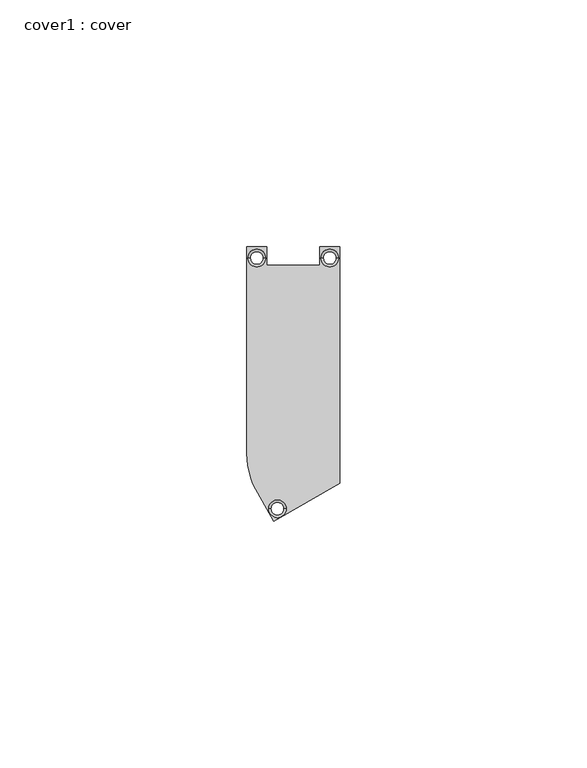
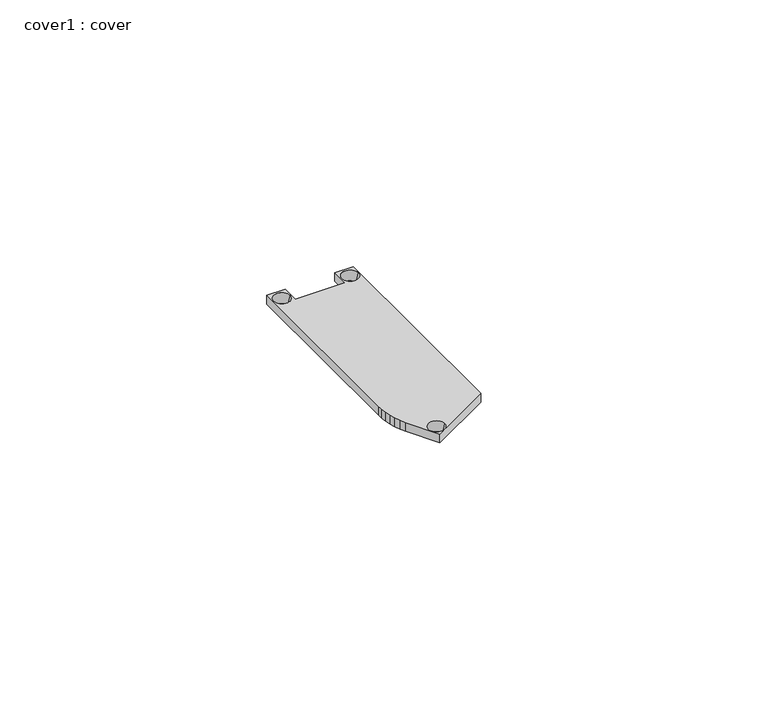
"""IFC4 building model written with IfcOpenShell, lengths in millimetres: proxy geometry, cover1 : cover."""

from ifc_helpers import new_model, si_unit, frame, origin, place, context, project, spatial, polyline, circle_curve, source, transform, mapped, element, save
from ifc_brep_helpers import plane_surface, revolved_surface, advanced_brep


def cover1_cover_a61f0212(model_context):
    return source(origin(), model_context, "Body", "AdvancedBrep", [
        advanced_brep(
        [(4738.4618953, 3578.6670305, 2.0), (4734.4613953, 3578.6670305, 2.0), (4734.4613953, 3574.9179905, 2.0), (4723.6816353, 3574.9179905, 2.0), (4723.6816353, 3578.6670305, 2.0), (4719.6811353, 3578.6670305, 2.0), (4719.6811353, 3536.8840305, 2.0), (4719.7370153, 3535.6191105, 2.0), (4719.8919553, 3534.3618105, 2.0), (4720.1383353, 3533.1222905, 2.0), (4720.4786953, 3531.9030905, 2.0), (4720.9079553, 3530.7118305, 2.0), (4721.4261153, 3529.5586705, 2.0), (4725.1243775, 3523.1530364, 2.0), (4738.4618953, 3530.8564939, 2.0), (4738.2616453, 3576.4165905, 2.0), (4734.6616453, 3576.4165905, 2.0), (4723.4801153, 3576.4165905, 2.0), (4719.8801153, 3576.4165905, 2.0), (4727.6343594, 3525.6369105, 2.0), (4724.0799311, 3525.6369105, 2.0), (4738.4618953, 3578.6670305, 0.0), (4738.4618953, 3530.8564939, 0.0), (4725.1243775, 3523.1530364, 0.0), (4721.4261153, 3529.5586705, 0.0), (4720.9079553, 3530.7118305, 0.0), (4720.4786953, 3531.9030905, 0.0), (4720.1383353, 3533.1222905, 0.0), (4719.8919553, 3534.3618105, 0.0), (4719.7370153, 3535.6191105, 0.0), (4719.6811353, 3536.8840305, 0.0), (4719.6811353, 3578.6670305, 0.0), (4723.6816353, 3578.6670305, 0.0), (4723.6816353, 3574.9179905, 0.0), (4734.4613953, 3574.9179905, 0.0), (4734.4613953, 3578.6670305, 0.0), (4735.1616453, 3576.4165905, 0.0), (4737.7616453, 3576.4165905, 0.0), (4720.3801153, 3576.4165905, 0.0), (4722.9801153, 3576.4165905, 0.0), (4724.5418919, 3525.6369105, 0.0), (4727.1723986, 3525.6369105, 0.0)],
        [
            (0, 1),
            (1, 2),
            (2, 3),
            (3, 4),
            (4, 5),
            (5, 6),
            (6, 7),
            (7, 8),
            (8, 9),
            (9, 10),
            (10, 11),
            (11, 12),
            (12, 13),
            (13, 14),
            (14, 0),
            (15, 16, circle_curve(frame((4736.4616453, 3576.4165905, 2.0), z_axis=(0.0, 0.0, -1.0), x_axis=(-1.0, 0.0, 0.0)), 1.8)),
            (16, 15, circle_curve(frame((4736.4616453, 3576.4165905, 2.0), z_axis=(0.0, 0.0, -1.0), x_axis=(1.0, 0.0, 0.0)), 1.8)),
            (17, 18, circle_curve(frame((4721.6801153, 3576.4165905, 2.0), z_axis=(0.0, 0.0, -1.0), x_axis=(-1.0, 0.0, 0.0)), 1.8)),
            (18, 17, circle_curve(frame((4721.6801153, 3576.4165905, 2.0), z_axis=(0.0, 0.0, -1.0), x_axis=(1.0, 0.0, 0.0)), 1.8)),
            (19, 20, circle_curve(frame((4725.8571453, 3525.6369105, 2.0), z_axis=(0.0, 0.0, -1.0), x_axis=(-1.0, 0.0, 0.0)), 1.7772142)),
            (20, 19, circle_curve(frame((4725.8571453, 3525.6369105, 2.0), z_axis=(0.0, 0.0, -1.0), x_axis=(1.0, 0.0, 0.0)), 1.7772142)),
            (21, 22),
            (22, 23),
            (23, 24),
            (24, 25),
            (25, 26),
            (26, 27),
            (27, 28),
            (28, 29),
            (29, 30),
            (30, 31),
            (31, 32),
            (32, 33),
            (33, 34),
            (34, 35),
            (35, 21),
            (36, 37, circle_curve(frame((4736.4616453, 3576.4165905, 0.0), z_axis=(0.0, 0.0, 1.0), x_axis=(-1.0, 0.0, 0.0)), 1.3)),
            (37, 36, circle_curve(frame((4736.4616453, 3576.4165905, 0.0), z_axis=(0.0, 0.0, 1.0), x_axis=(1.0, 0.0, 0.0)), 1.3)),
            (38, 39, circle_curve(frame((4721.6801153, 3576.4165905, 0.0), z_axis=(0.0, 0.0, 1.0), x_axis=(-1.0, 0.0, 0.0)), 1.3)),
            (39, 38, circle_curve(frame((4721.6801153, 3576.4165905, 0.0), z_axis=(0.0, 0.0, 1.0), x_axis=(1.0, 0.0, 0.0)), 1.3)),
            (40, 41, circle_curve(frame((4725.8571453, 3525.6369105, 0.0), z_axis=(0.0, 0.0, 1.0), x_axis=(-1.0, 0.0, 0.0)), 1.3152534)),
            (41, 40, circle_curve(frame((4725.8571453, 3525.6369105, 0.0), z_axis=(0.0, 0.0, 1.0), x_axis=(1.0, 0.0, 0.0)), 1.3152534)),
            (14, 22),
            (21, 0),
            (13, 23),
            (12, 24),
            (5, 31),
            (30, 6),
            (11, 25),
            (10, 26),
            (9, 27),
            (8, 28),
            (7, 29),
            (4, 32),
            (36, 16),
            (15, 37),
            (38, 18),
            (17, 39),
            (40, 20),
            (19, 41),
            (3, 33),
            (2, 34),
            (1, 35),
        ],
        [
            plane_surface(frame((4734.4613953, 3578.6670305, 2.0), z_axis=(0.0, 0.0, 1.0), x_axis=(-1.0, 0.0, 0.0))),
            plane_surface(frame((4734.4613953, 3578.6670305, 0.0), z_axis=(0.0, 0.0, -1.0), x_axis=(1.0, 0.0, 0.0))),
            plane_surface(frame((4738.4618953, 3530.8564939, 2.0), z_axis=(1.0, 0.0, 0.0), x_axis=(0.0, 0.0, -1.0))),
            plane_surface(frame((4725.1243775, 3523.1530364, 2.0), z_axis=(0.5001479267947538, -0.8659399813629751, 0.0), x_axis=(0.0, 0.0, -1.0))),
            plane_surface(frame((4721.4261153, 3529.5586705, 2.0), z_axis=(-0.8660272939548952, -0.49999672611444335, 0.0), x_axis=(0.0, 0.0, -1.0))),
            plane_surface(frame((4719.6811353, 3578.6670305, 2.0), z_axis=(-1.0, 0.0, 0.0), x_axis=(0.0, 0.0, -1.0))),
            plane_surface(frame((4720.9079553, 3530.7118305, 2.0), z_axis=(-0.91214692510674, -0.40986337603928397, 0.0), x_axis=(0.0, 0.0, -1.0))),
            plane_surface(frame((4720.4786953, 3531.9030905, 2.0), z_axis=(-0.9407850831608502, -0.3390035800725891, 0.0), x_axis=(0.0, 0.0, -1.0))),
            plane_surface(frame((4720.1383353, 3533.1222905, 2.0), z_axis=(-0.9631721335643817, -0.26888555395379093, 0.0), x_axis=(0.0, 0.0, -1.0))),
            plane_surface(frame((4719.8919553, 3534.3618105, 2.0), z_axis=(-0.9808118970912181, -0.19495646315094542, 0.0), x_axis=(0.0, 0.0, -1.0))),
            plane_surface(frame((4719.7370153, 3535.6191105, 2.0), z_axis=(-0.9924922999614717, -0.12230713191465294, 0.0), x_axis=(0.0, 0.0, -1.0))),
            plane_surface(frame((4719.6811353, 3536.8840305, 2.0), z_axis=(-0.9990256352193916, -0.04413366260000536, 0.0), x_axis=(0.0, 0.0, -1.0))),
            plane_surface(frame((4723.6816353, 3578.6670305, 2.0), z_axis=(0.0, 1.0, 0.0), x_axis=(0.0, 0.0, -1.0))),
            revolved_surface(polyline([(4734.6616453, 3576.4165905, 2.0), (4735.1616453, 3576.4165905, 0.0)]), (4736.4616453, 3576.4165905, -5.2), (0.0, 0.0, 1.0)),
            revolved_surface(polyline([(4719.8801153, 3576.4165905, 2.0), (4720.3801153, 3576.4165905, 0.0)]), (4721.6801153, 3576.4165905, -5.2), (0.0, 0.0, 1.0)),
            revolved_surface(polyline([(4724.0799311, 3525.6369105, 2.0), (4724.5418919125095, 3525.6369105, 0.0)]), (4725.8571453, 3525.6369105, -5.6942206), (0.0, 0.0, 1.0)),
            plane_surface(frame((4723.6816353, 3574.9179905, 2.0), z_axis=(1.0, 0.0, 0.0), x_axis=(0.0, 0.0, -1.0))),
            plane_surface(frame((4734.4613953, 3574.9179905, 2.0), z_axis=(0.0, 1.0, 0.0), x_axis=(0.0, 0.0, -1.0))),
            plane_surface(frame((4734.4613953, 3578.6670305, 2.0), z_axis=(-1.0, 0.0, 0.0), x_axis=(0.0, 0.0, -1.0))),
            plane_surface(frame((4738.4618953, 3578.6670305, 2.0), z_axis=(0.0, 1.0, 0.0), x_axis=(0.0, 0.0, -1.0))),
        ],
        [
            (0, [[1, 2, 3, 4, 5, 6, 7, 8, 9, 10, 11, 12, 13, 14, 15], [16, 17], [18, 19], [20, 21]]),
            (1, [[22, 23, 24, 25, 26, 27, 28, 29, 30, 31, 32, 33, 34, 35, 36], [37, 38], [39, 40], [41, 42]]),
            (2, [[-15, 43, -22, 44]]),
            (3, [[-14, 45, -23, -43]]),
            (4, [[-13, 46, -24, -45]]),
            (5, [[-6, 47, -31, 48]]),
            (6, [[-12, 49, -25, -46]]),
            (7, [[-11, 50, -26, -49]]),
            (8, [[-10, 51, -27, -50]]),
            (9, [[-9, 52, -28, -51]]),
            (10, [[-8, 53, -29, -52]]),
            (11, [[-7, -48, -30, -53]]),
            (12, [[-5, 54, -32, -47]]),
            (13, [[55, -16, 56, -37]]),
            (13, [[-55, -38, -56, -17]]),
            (14, [[57, -18, 58, -39]]),
            (14, [[-57, -40, -58, -19]]),
            (15, [[59, -20, 60, -41]]),
            (15, [[-59, -42, -60, -21]]),
            (16, [[-4, 61, -33, -54]]),
            (17, [[-3, 62, -34, -61]]),
            (18, [[-2, 63, -35, -62]]),
            (19, [[-1, -44, -36, -63]]),
        ],
    ),
    ])


if __name__ == "__main__":
    model = new_model("IFC4")
    model_context = context("Model", 3, world=origin())
    ifc_project = project(units=[si_unit("LENGTHUNIT", "METRE", prefix="MILLI")], contexts=[model_context])
    site = spatial("IfcSite", under=ifc_project)
    building = spatial("IfcBuilding", under=site)
    placement = place(None, origin())
    cover1_cover_shape = cover1_cover_a61f0212(model_context)
    element("IfcBuildingElementProxy", 1, Name="cover1 : cover", ObjectType="cover1 : cover", at=placement, inside=building, context=model_context, shape_type="MappedRepresentation", body=[
        mapped(cover1_cover_shape, transform((0.0, 0.0, 0.0), x_axis=(1.0, 0.0, 0.0), y_axis=(0.0, 1.0, 0.0), z_axis=(0.0, 0.0, 1.0))),
    ])
    save(model, "model.ifc")

# Revit data of these elements
# Project information
#   Data de emissão do projeto = "Data de emissão"
#   Status do projeto = "Status do projeto"
#   Nome do cliente = "Proprietário"
#   Endereço do projeto = "Insira aqui o endereço"
#   Nome do projeto = "Nome do projeto"
#   Número do projeto = "0001"
